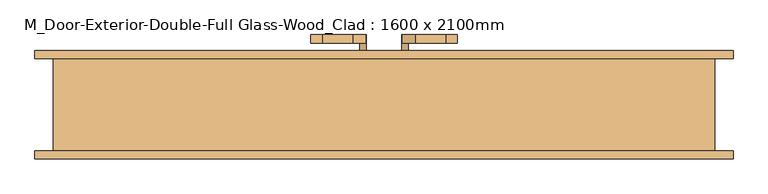
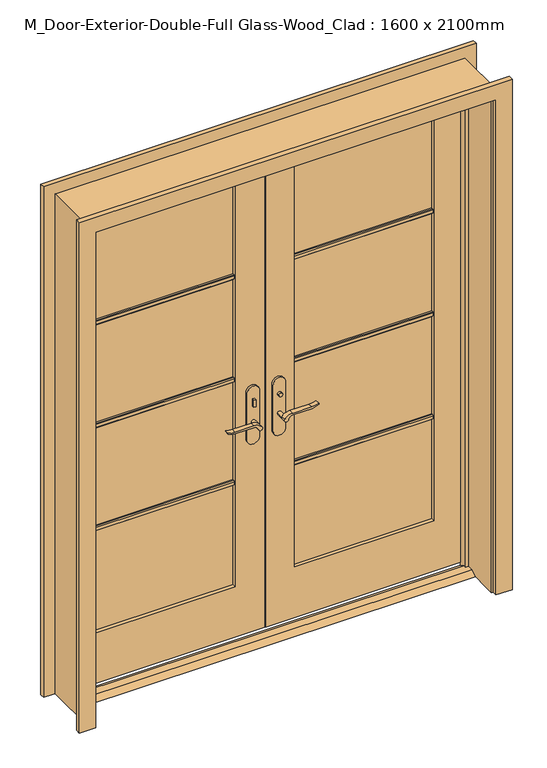
"""IFC4 building model written with IfcOpenShell, lengths in millimetres: door geometry, M_Door-Exterior-Double-Full Glass-Wood_Clad : 1600 x 2100mm."""

from ifc_helpers import new_model, si_unit, point, frame, frame_2d, origin, place, context, project, spatial, polyline, circle_curve, trimmed, segment, composite_curve, outline, extrude, faceted_brep, source, transform, mapped, element, save


def m_door_exterior_double_full_glass_wood_clad_1600_x_2100mm_56e3e291(model_context):
    return source(origin(), model_context, "Body", "SolidModel", [
        extrude(outline(polyline([(18.975, 15.0), (53.975, 15.0), (79.375, 0.0), (-6.425, 0.0), (18.975, 15.0)])), frame((-800.0, 0.0, 0.0), z_axis=(1.0, 0.0, 0.0), x_axis=(0.0, 1.0, 0.0)), (0.0, 0.0, 1.0), 1600.0),
        extrude(outline(polyline([(-47.4019111, 56.825), (-57.4019111, 56.825), (-57.4019111, 66.825), (-47.4019111, 66.825), (-47.4019111, 56.825)])), frame((0.0, 0.0, 981.9), z_axis=(0.0, 0.0, 1.0), x_axis=(1.0, 0.0, 0.0)), (0.0, 0.0, 1.0), 30.0),
        extrude(outline(composite_curve([segment(trimmed(circle_curve(frame_2d((996.9, -52.4019111)), 8.0), [point((996.9, -60.4019111))], [point((996.9, -44.4019111))], False, "CARTESIAN"), True, "CONTINUOUS"), segment(trimmed(circle_curve(frame_2d((996.9, -52.4019111)), 8.0), [point((996.9, -44.4019111))], [point((996.9, -60.4019111))], False, "CARTESIAN"), True, "CONTINUOUS")], self_intersect=False)), frame((0.0, 121.825, 0.0), z_axis=(0.0, 1.0, 0.0), x_axis=(0.0, 0.0, 1.0)), (0.0, 0.0, 1.0), 10.0),
        extrude(outline(composite_curve([segment(trimmed(circle_curve(frame_2d((897.1555521, -76.0694241)), 37.2832219), [point((919.0523287, -45.8937749))], [point((934.4, -77.7693445))], False, "CARTESIAN"), True, "CONTINUOUS"), segment(polyline([(934.4, -77.7693445), (934.4, -154.045502)]), True, "CONTINUOUS"), segment(trimmed(circle_curve(frame_2d((1017.6850638, -153.9791202)), 83.2850902), [point((934.4, -154.045502))], [point((939.4, -182.4019111))], True, "CARTESIAN"), True, "CONTINUOUS"), segment(polyline([(939.4, -182.4019111), (936.6135558, -182.4019111)]), True, "CONTINUOUS"), segment(trimmed(circle_curve(frame_2d((986.6709207, -150.4622499)), 59.3791355), [point((936.6135558, -182.4019111))], [point((927.4, -154.045502))], False, "CARTESIAN"), True, "CONTINUOUS"), segment(polyline([(927.4, -154.045502), (927.4, -77.7881013)]), True, "CONTINUOUS"), segment(trimmed(circle_curve(frame_2d((909.2738613, -77.7881013)), 18.1261387), [point((927.4, -77.7881013))], [point((914.4, -60.4019111))], True, "CARTESIAN"), True, "CONTINUOUS"), segment(trimmed(circle_curve(frame_2d((914.4, -52.4019111)), 8.0), [point((914.4, -60.4019111))], [point((919.0523287, -45.8937749))], False, "CARTESIAN"), True, "CONTINUOUS")], self_intersect=False)), frame((0.0, 16.825, 0.0), z_axis=(0.0, 1.0, 0.0), x_axis=(0.0, 0.0, 1.0)), (0.0, 0.0, 1.0), 20.0),
        extrude(outline(composite_curve([segment(trimmed(circle_curve(frame_2d((914.4, -52.4019111)), 8.0), [point((914.3999903, -60.4019111))], [point((919.0523287, -45.8937749))], False, "CARTESIAN"), True, "CONTINUOUS"), segment(trimmed(circle_curve(frame_2d((897.1555521, -76.0694241)), 37.2832219), [point((919.0523287, -45.8937749))], [point((934.4, -77.7693445))], False, "CARTESIAN"), True, "CONTINUOUS"), segment(polyline([(934.4, -77.7693445), (934.4, -154.045502)]), True, "CONTINUOUS"), segment(trimmed(circle_curve(frame_2d((1017.6850638, -153.9791202)), 83.2850902), [point((934.4, -154.045502))], [point((939.4, -182.4019111))], True, "CARTESIAN"), True, "CONTINUOUS"), segment(polyline([(939.4, -182.4019111), (936.6135558, -182.4019111)]), True, "CONTINUOUS"), segment(trimmed(circle_curve(frame_2d((986.6709207, -150.4622499)), 59.3791355), [point((936.6135558, -182.4019111))], [point((927.4, -154.045502))], False, "CARTESIAN"), True, "CONTINUOUS"), segment(polyline([(927.4, -154.045502), (927.4, -77.788099)]), True, "CONTINUOUS"), segment(trimmed(circle_curve(frame_2d((909.2738682, -77.788099)), 18.1261318), [point((927.4, -77.788099))], [point((914.3999903, -60.4019111))], True, "CARTESIAN"), True, "CONTINUOUS")], self_intersect=False)), frame((0.0, 151.825, 0.0), z_axis=(0.0, 1.0, 0.0), x_axis=(0.0, 0.0, 1.0)), (0.0, 0.0, 1.0), 20.0),
        extrude(outline(composite_curve([segment(trimmed(circle_curve(frame_2d((914.4, -52.4019111)), 8.0), [point((914.4, -60.4019111))], [point((914.4, -44.4019111))], False, "CARTESIAN"), True, "CONTINUOUS"), segment(trimmed(circle_curve(frame_2d((914.4, -52.4019111)), 8.0), [point((914.4, -44.4019111))], [point((914.4, -60.4019111))], False, "CARTESIAN"), True, "CONTINUOUS")], self_intersect=False)), frame((0.0, 36.825, 0.0), z_axis=(0.0, 1.0, 0.0), x_axis=(0.0, 0.0, 1.0)), (0.0, 0.0, 1.0), 30.0),
        extrude(outline(composite_curve([segment(trimmed(circle_curve(frame_2d((914.4, -52.4019111)), 8.0), [point((914.4, -60.4019111))], [point((914.4, -44.4019111))], False, "CARTESIAN"), True, "CONTINUOUS"), segment(trimmed(circle_curve(frame_2d((914.4, -52.4019111)), 8.0), [point((914.4, -44.4019111))], [point((914.4, -60.4019111))], False, "CARTESIAN"), True, "CONTINUOUS")], self_intersect=False)), frame((0.0, 121.825, 0.0), z_axis=(0.0, 1.0, 0.0), x_axis=(0.0, 0.0, 1.0)), (0.0, 0.0, 1.0), 30.0),
        extrude(outline(composite_curve([segment(polyline([(844.4, -27.4019111), (1039.4, -27.4019111)]), True, "CONTINUOUS"), segment(trimmed(circle_curve(frame_2d((1039.4, -52.4019111)), 25.0), [point((1039.4, -27.4019111))], [point((1039.4, -77.4019111))], False, "CARTESIAN"), True, "CONTINUOUS"), segment(polyline([(1039.4, -77.4019111), (844.4, -77.4019111)]), True, "CONTINUOUS"), segment(trimmed(circle_curve(frame_2d((844.4, -52.4019111)), 25.0), [point((844.4, -77.4019111))], [point((844.4, -27.4019111))], False, "CARTESIAN"), True, "CONTINUOUS")], self_intersect=False)), frame((0.0, 66.825, 0.0), z_axis=(0.0, 1.0, 0.0), x_axis=(0.0, 0.0, 1.0)), (0.0, 0.0, 1.0), 10.0),
        extrude(outline(composite_curve([segment(polyline([(844.4, -27.4019111), (1039.4, -27.4019111)]), True, "CONTINUOUS"), segment(trimmed(circle_curve(frame_2d((1039.4, -52.4019111)), 25.0), [point((1039.4, -27.4019111))], [point((1039.4, -77.4019111))], False, "CARTESIAN"), True, "CONTINUOUS"), segment(polyline([(1039.4, -77.4019111), (844.4, -77.4019111)]), True, "CONTINUOUS"), segment(trimmed(circle_curve(frame_2d((844.4, -52.4019111)), 25.0), [point((844.4, -77.4019111))], [point((844.4, -27.4019111))], False, "CARTESIAN"), True, "CONTINUOUS")], self_intersect=False)), frame((0.0, 111.825, 0.0), z_axis=(0.0, 1.0, 0.0), x_axis=(0.0, 0.0, 1.0)), (0.0, 0.0, 1.0), 10.0),
        extrude(outline(polyline([(47.3875, 131.825), (57.3875, 131.825), (57.3875, 121.825), (47.3875, 121.825), (47.3875, 131.825)])), frame((0.0, 0.0, 981.9), z_axis=(0.0, 0.0, 1.0), x_axis=(1.0, 0.0, 0.0)), (0.0, 0.0, 1.0), 30.0),
        extrude(outline(composite_curve([segment(trimmed(circle_curve(frame_2d((996.9, 52.3875)), 8.0), [point((996.9, 60.3875))], [point((996.9, 44.3875))], False, "CARTESIAN"), True, "CONTINUOUS"), segment(trimmed(circle_curve(frame_2d((996.9, 52.3875)), 8.0), [point((996.9, 44.3875))], [point((996.9, 60.3875))], False, "CARTESIAN"), True, "CONTINUOUS")], self_intersect=False)), frame((0.0, 56.825, 0.0), z_axis=(0.0, 1.0, 0.0), x_axis=(0.0, 0.0, 1.0)), (0.0, 0.0, 1.0), 10.0),
        extrude(outline(composite_curve([segment(trimmed(circle_curve(frame_2d((914.4, 52.3875)), 8.0), [point((919.0523287, 45.8793637))], [point((914.4, 60.3875))], False, "CARTESIAN"), True, "CONTINUOUS"), segment(trimmed(circle_curve(frame_2d((909.2738613, 77.7736901)), 18.1261387), [point((914.4, 60.3875))], [point((927.4, 77.7736901))], True, "CARTESIAN"), True, "CONTINUOUS"), segment(polyline([(927.4, 77.7736901), (927.4, 154.0310909)]), True, "CONTINUOUS"), segment(trimmed(circle_curve(frame_2d((986.6709207, 150.4478388)), 59.3791355), [point((927.4, 154.0310909))], [point((936.6135558, 182.3875))], False, "CARTESIAN"), True, "CONTINUOUS"), segment(polyline([(936.6135558, 182.3875), (939.4, 182.3875)]), True, "CONTINUOUS"), segment(trimmed(circle_curve(frame_2d((1017.6850638, 153.9647091)), 83.2850902), [point((939.4, 182.3875))], [point((934.4, 154.0310909))], True, "CARTESIAN"), True, "CONTINUOUS"), segment(polyline([(934.4, 154.0310909), (934.4, 77.7549333)]), True, "CONTINUOUS"), segment(trimmed(circle_curve(frame_2d((897.1555521, 76.0550129)), 37.2832219), [point((934.4, 77.7549333))], [point((919.0523287, 45.8793637))], False, "CARTESIAN"), True, "CONTINUOUS")], self_intersect=False)), frame((0.0, 151.825, 0.0), z_axis=(0.0, 1.0, 0.0), x_axis=(0.0, 0.0, 1.0)), (0.0, 0.0, 1.0), 20.0),
        extrude(outline(composite_curve([segment(trimmed(circle_curve(frame_2d((909.2738682, 77.7736878)), 18.1261318), [point((914.3999903, 60.3875))], [point((927.4, 77.7736878))], True, "CARTESIAN"), True, "CONTINUOUS"), segment(polyline([(927.4, 77.7736878), (927.4, 154.0310909)]), True, "CONTINUOUS"), segment(trimmed(circle_curve(frame_2d((986.6709207, 150.4478388)), 59.3791355), [point((927.4, 154.0310909))], [point((936.6135558, 182.3875))], False, "CARTESIAN"), True, "CONTINUOUS"), segment(polyline([(936.6135558, 182.3875), (939.4, 182.3875)]), True, "CONTINUOUS"), segment(trimmed(circle_curve(frame_2d((1017.6850638, 153.9647091)), 83.2850902), [point((939.4, 182.3875))], [point((934.4, 154.0310909))], True, "CARTESIAN"), True, "CONTINUOUS"), segment(polyline([(934.4, 154.0310909), (934.4, 77.7549333)]), True, "CONTINUOUS"), segment(trimmed(circle_curve(frame_2d((897.1555521, 76.0550129)), 37.2832219), [point((934.4, 77.7549333))], [point((919.0523287, 45.8793637))], False, "CARTESIAN"), True, "CONTINUOUS"), segment(trimmed(circle_curve(frame_2d((914.4, 52.3875)), 8.0), [point((919.0523287, 45.8793637))], [point((914.3999903, 60.3875))], False, "CARTESIAN"), True, "CONTINUOUS")], self_intersect=False)), frame((0.0, 16.825, 0.0), z_axis=(0.0, 1.0, 0.0), x_axis=(0.0, 0.0, 1.0)), (0.0, 0.0, 1.0), 20.0),
        extrude(outline(composite_curve([segment(trimmed(circle_curve(frame_2d((914.4, 52.3875)), 8.0), [point((914.4, 60.3875))], [point((914.4, 44.3875))], False, "CARTESIAN"), True, "CONTINUOUS"), segment(trimmed(circle_curve(frame_2d((914.4, 52.3875)), 8.0), [point((914.4, 44.3875))], [point((914.4, 60.3875))], False, "CARTESIAN"), True, "CONTINUOUS")], self_intersect=False)), frame((0.0, 121.825, 0.0), z_axis=(0.0, 1.0, 0.0), x_axis=(0.0, 0.0, 1.0)), (0.0, 0.0, 1.0), 30.0),
        extrude(outline(composite_curve([segment(trimmed(circle_curve(frame_2d((914.4, 52.3875)), 8.0), [point((914.4, 60.3875))], [point((914.4, 44.3875))], False, "CARTESIAN"), True, "CONTINUOUS"), segment(trimmed(circle_curve(frame_2d((914.4, 52.3875)), 8.0), [point((914.4, 44.3875))], [point((914.4, 60.3875))], False, "CARTESIAN"), True, "CONTINUOUS")], self_intersect=False)), frame((0.0, 36.825, 0.0), z_axis=(0.0, 1.0, 0.0), x_axis=(0.0, 0.0, 1.0)), (0.0, 0.0, 1.0), 30.0),
        extrude(outline(composite_curve([segment(trimmed(circle_curve(frame_2d((844.4, 52.3875)), 25.0), [point((844.4, 27.3875))], [point((844.4, 77.3875))], False, "CARTESIAN"), True, "CONTINUOUS"), segment(polyline([(844.4, 77.3875), (1039.4, 77.3875)]), True, "CONTINUOUS"), segment(trimmed(circle_curve(frame_2d((1039.4, 52.3875)), 25.0), [point((1039.4, 77.3875))], [point((1039.4, 27.3875))], False, "CARTESIAN"), True, "CONTINUOUS"), segment(polyline([(1039.4, 27.3875), (844.4, 27.3875)]), True, "CONTINUOUS")], self_intersect=False)), frame((0.0, 111.825, 0.0), z_axis=(0.0, 1.0, 0.0), x_axis=(0.0, 0.0, 1.0)), (0.0, 0.0, 1.0), 10.0),
        extrude(outline(composite_curve([segment(trimmed(circle_curve(frame_2d((844.4, 52.3875)), 25.0), [point((844.4, 27.3875))], [point((844.4, 77.3875))], False, "CARTESIAN"), True, "CONTINUOUS"), segment(polyline([(844.4, 77.3875), (1039.4, 77.3875)]), True, "CONTINUOUS"), segment(trimmed(circle_curve(frame_2d((1039.4, 52.3875)), 25.0), [point((1039.4, 77.3875))], [point((1039.4, 27.3875))], False, "CARTESIAN"), True, "CONTINUOUS"), segment(polyline([(1039.4, 27.3875), (844.4, 27.3875)]), True, "CONTINUOUS")], self_intersect=False)), frame((0.0, 66.825, 0.0), z_axis=(0.0, 1.0, 0.0), x_axis=(0.0, 0.0, 1.0)), (0.0, 0.0, 1.0), 10.0),
        extrude(outline(polyline([(90.825, 1552.025), (90.825, 1532.975), (84.475, 1532.975), (81.3, 1536.15), (81.3, 1548.85), (84.475, 1552.025), (90.825, 1552.025)])), frame((120.0, 0.0, 0.0), z_axis=(1.0, 0.0, 0.0), x_axis=(0.0, 1.0, 0.0)), (0.0, 0.0, 1.0), 560.0),
        extrude(outline(polyline([(90.825, 1114.525), (90.825, 1095.475), (84.475, 1095.475), (81.3, 1098.65), (81.3, 1111.35), (84.475, 1114.525), (90.825, 1114.525)])), frame((120.0, 0.0, 0.0), z_axis=(1.0, 0.0, 0.0), x_axis=(0.0, 1.0, 0.0)), (0.0, 0.0, 1.0), 560.0),
        extrude(outline(polyline([(90.825, 677.025), (90.825, 657.975), (84.475, 657.975), (81.3, 661.15), (81.3, 673.85), (84.475, 677.025), (90.825, 677.025)])), frame((120.0, 0.0, 0.0), z_axis=(1.0, 0.0, 0.0), x_axis=(0.0, 1.0, 0.0)), (0.0, 0.0, 1.0), 560.0),
        extrude(outline(polyline([(97.825, 1552.025), (104.175, 1552.025), (107.35, 1548.85), (107.35, 1536.15), (104.175, 1532.975), (97.825, 1532.975), (97.825, 1552.025)])), frame((-680.0, 0.0, 0.0), z_axis=(1.0, 0.0, 0.0), x_axis=(0.0, 1.0, 0.0)), (0.0, 0.0, 1.0), 560.0),
        extrude(outline(polyline([(97.825, 1114.525), (104.175, 1114.525), (107.35, 1111.35), (107.35, 1098.65), (104.175, 1095.475), (97.825, 1095.475), (97.825, 1114.525)])), frame((-680.0, 0.0, 0.0), z_axis=(1.0, 0.0, 0.0), x_axis=(0.0, 1.0, 0.0)), (0.0, 0.0, 1.0), 560.0),
        extrude(outline(polyline([(97.825, 677.025), (104.175, 677.025), (107.35, 673.85), (107.35, 661.15), (104.175, 657.975), (97.825, 657.975), (97.825, 677.025)])), frame((-680.0, 0.0, 0.0), z_axis=(1.0, 0.0, 0.0), x_axis=(0.0, 1.0, 0.0)), (0.0, 0.0, 1.0), 560.0),
        extrude(outline(polyline([(97.825, 1552.025), (104.175, 1552.025), (107.35, 1548.85), (107.35, 1536.15), (104.175, 1532.975), (97.825, 1532.975), (97.825, 1552.025)])), frame((120.0, 0.0, 0.0), z_axis=(1.0, 0.0, 0.0), x_axis=(0.0, 1.0, 0.0)), (0.0, 0.0, 1.0), 560.0),
        extrude(outline(polyline([(97.825, 1114.525), (104.175, 1114.525), (107.35, 1111.35), (107.35, 1098.65), (104.175, 1095.475), (97.825, 1095.475), (97.825, 1114.525)])), frame((120.0, 0.0, 0.0), z_axis=(1.0, 0.0, 0.0), x_axis=(0.0, 1.0, 0.0)), (0.0, 0.0, 1.0), 560.0),
        extrude(outline(polyline([(97.825, 677.025), (104.175, 677.025), (107.35, 673.85), (107.35, 661.15), (104.175, 657.975), (97.825, 657.975), (97.825, 677.025)])), frame((120.0, 0.0, 0.0), z_axis=(1.0, 0.0, 0.0), x_axis=(0.0, 1.0, 0.0)), (0.0, 0.0, 1.0), 560.0),
        extrude(outline(polyline([(90.825, 1552.025), (90.825, 1532.975), (84.475, 1532.975), (81.3, 1536.15), (81.3, 1548.85), (84.475, 1552.025), (90.825, 1552.025)])), frame((-680.0, 0.0, 0.0), z_axis=(1.0, 0.0, 0.0), x_axis=(0.0, 1.0, 0.0)), (0.0, 0.0, 1.0), 560.0),
        extrude(outline(polyline([(90.825, 1114.525), (90.825, 1095.475), (84.475, 1095.475), (81.3, 1098.65), (81.3, 1111.35), (84.475, 1114.525), (90.825, 1114.525)])), frame((-680.0, 0.0, 0.0), z_axis=(1.0, 0.0, 0.0), x_axis=(0.0, 1.0, 0.0)), (0.0, 0.0, 1.0), 560.0),
        extrude(outline(polyline([(90.825, 677.025), (90.825, 657.975), (84.475, 657.975), (81.3, 661.15), (81.3, 673.85), (84.475, 677.025), (90.825, 677.025)])), frame((-680.0, 0.0, 0.0), z_axis=(1.0, 0.0, 0.0), x_axis=(0.0, 1.0, 0.0)), (0.0, 0.0, 1.0), 560.0),
        extrude(outline(polyline([(0.0, 806.35), (0.0, 871.35), (2171.35, 871.35), (2171.35, -871.35), (0.0, -871.35), (0.0, -806.35), (2106.35, -806.35), (2106.35, 806.35), (0.0, 806.35)])), frame((0.0, 111.825, 0.0), z_axis=(0.0, 1.0, 0.0), x_axis=(0.0, 0.0, 1.0)), (0.0, 0.0, 1.0), 20.0),
        extrude(outline(polyline([(0.0, 806.35), (0.0, 871.35), (2171.35, 871.35), (2171.35, -871.35), (0.0, -871.35), (0.0, -806.35), (2106.35, -806.35), (2106.35, 806.35), (0.0, 806.35)])), frame((0.0, -138.175, 0.0), z_axis=(0.0, 1.0, 0.0), x_axis=(0.0, 0.0, 1.0)), (0.0, 0.0, 1.0), 20.0),
        extrude(outline(polyline([(15.0, 800.0), (2100.0, 800.0), (2100.0, 1.5875), (15.0, 1.5875), (15.0, 800.0)]), holes=[polyline([(1980.0, 120.0), (1980.0, 680.0), (230.0, 680.0), (230.0, 120.0), (1980.0, 120.0)])]), frame((0.0, 76.825, 0.0), z_axis=(0.0, 1.0, 0.0), x_axis=(0.0, 0.0, 1.0)), (0.0, 0.0, 1.0), 35.0),
        extrude(outline(polyline([(2100.0, -800.0), (15.0, -800.0), (15.0, -1.6019111), (2100.0, -1.6019111), (2100.0, -800.0)]), holes=[polyline([(230.0, -680.0), (1980.0, -680.0), (1980.0, -120.0), (230.0, -120.0), (230.0, -680.0)])]), frame((0.0, 76.825, 0.0), z_axis=(0.0, 1.0, 0.0), x_axis=(0.0, 0.0, 1.0)), (0.0, 0.0, 1.0), 35.0),
        faceted_brep([(825.0, 111.825, 0.0), (825.0, -118.175, 0.0), (800.0, -118.175, 0.0), (800.0, 41.9, 0.0), (787.3, 41.9, 0.0), (787.3, 76.825, 0.0), (800.0, 76.825, 0.0), (800.0, 111.825, 0.0), (825.0, 111.825, 2125.0), (825.0, -118.175, 2125.0), (-825.0, -118.175, 2125.0), (-825.0, -118.175, 0.0), (-800.0, -118.175, 0.0), (-800.0, -118.175, 2100.0), (800.0, -118.175, 2100.0), (800.0, 41.9, 2100.0), (-800.0, 41.9, 2100.0), (-800.0, 41.9, 0.0), (-787.3, 41.9, 0.0), (-787.3, 41.9, 2087.3), (787.3, 41.9, 2087.3), (787.3, 76.825, 2087.3), (1.5875, 76.825, 2087.3), (-1.6019111, 76.825, 2087.3), (-787.3, 76.825, 2087.3), (-787.3, 76.825, 0.0), (-800.0, 76.825, 0.0), (-800.0, 76.825, 2100.0), (-1.6019111, 76.825, 2100.0), (1.5875, 76.825, 2100.0), (800.0, 76.825, 2100.0), (800.0, 111.825, 2100.0), (1.5875, 111.825, 2100.0), (-1.6019111, 111.825, 2100.0), (-800.0, 111.825, 2100.0), (-800.0, 111.825, 0.0), (-825.0, 111.825, 0.0), (-825.0, 111.825, 2125.0)], [[[0, 1, 2, 3, 4, 5, 6, 7]], [[1, 0, 8, 9]], [[2, 1, 9, 10, 11, 12, 13, 14]], [[3, 2, 14, 15]], [[4, 3, 15, 16, 17, 18, 19, 20]], [[5, 4, 20, 21]], [[6, 5, 21, 22, 23, 24, 25, 26, 27, 28, 29, 30]], [[7, 6, 30, 31]], [[0, 7, 31, 32, 33, 34, 35, 36, 37, 8]], [[9, 8, 37, 10]], [[14, 13, 16, 15]], [[20, 19, 24, 23, 22, 21]], [[31, 30, 29, 28, 27, 34, 33, 32]], [[12, 11, 36, 35, 26, 25, 18, 17]], [[11, 10, 37, 36]], [[13, 12, 17, 16]], [[19, 18, 25, 24]], [[27, 26, 35, 34]]]),
        extrude(outline(polyline([(680.0, 90.825), (120.0, 90.825), (120.0, 97.825), (680.0, 97.825), (680.0, 90.825)])), frame((0.0, 0.0, 230.0), z_axis=(0.0, 0.0, 1.0), x_axis=(1.0, 0.0, 0.0)), (0.0, 0.0, 1.0), 1750.0),
        extrude(outline(polyline([(-120.0, 90.825), (-680.0, 90.825), (-680.0, 97.825), (-120.0, 97.825), (-120.0, 90.825)])), frame((0.0, 0.0, 230.0), z_axis=(0.0, 0.0, 1.0), x_axis=(1.0, 0.0, 0.0)), (0.0, 0.0, 1.0), 1750.0),
    ])


if __name__ == "__main__":
    model = new_model("IFC4")
    model_context = context("Model", 3, world=origin())
    ifc_project = project(units=[si_unit("LENGTHUNIT", "METRE", prefix="MILLI")], contexts=[model_context])
    site = spatial("IfcSite", under=ifc_project)
    building = spatial("IfcBuilding", under=site)
    placement = place(None, origin())
    m_door_exterior_double_full_glass_wood_clad_1600_x_2100mm_shape = m_door_exterior_double_full_glass_wood_clad_1600_x_2100mm_56e3e291(model_context)
    element("IfcDoor", 1, ObjectType="M_Door-Exterior-Double-Full Glass-Wood_Clad : 1600 x 2100mm", at=placement, inside=building, context=model_context, shape_type="MappedRepresentation", body=[
        mapped(m_door_exterior_double_full_glass_wood_clad_1600_x_2100mm_shape, transform((0.0, 0.0, 0.0), x_axis=(1.0, 0.0, 0.0), y_axis=(0.0, 1.0, 0.0), z_axis=(0.0, 0.0, 1.0))),
    ])
    save(model, "model.ifc")

# Revit data of these elements
# Type "M_Door-Exterior-Double-Full Glass-Wood_Clad : 1600 x 2100mm"
#   Type Mark = "41"
#   Assembly Code = "B2030100"
#   Analytic Construction = "French door, wood frame with double glass"
#   Top Rail = 12 cm
#   Threshold Offset [instance default] = 1.5 cm
#   Thickness = 3.5 cm
#   Thermal Resistance (R) = 0.337392 (m²·K)/W
#   Swing Angle [instance default] = 90.00°
#   Stiles = 12 cm
#   Rough Width = 165 cm
#   Rough Height = 212.5 cm
#   Panel Width = 80 cm
#   Door Offset [instance default] = 0 cm
#   Height = 210 cm
#   Width = 160 cm
#   Heat Transfer Coefficient (U) = 2.96405 W/(m²·K)
#   Bottom Rail = 23 cm
#   Exterior Trim [instance default] = yes
#   Threshold [instance default] = yes
#   Show Grill [instance default] = yes
#   Function = 1
#   Trim Material = Cherry
#   Threshold Material = Cherry
#   Panel Material = Cherry
#   Glazing = Glass
#   Frame Material = Cherry
#   Door Handle Material = Aluminum
#   Visual Light Transmittance = 0
#   Solar Heat Gain Coefficient = 0
#   Wall Closure = (empty or 0)
#   Construction Type = (empty or 0)
# Element 1 (IfcDoor, "M_Door-Exterior-Double-Full Glass-Wood_Clad : 1600 x 2100mm")
#   Materials on its faces: "Cherry", "Aluminum", "Glass"
# Materials
#   "Cherry": class "Wood", colour RGB 226 177 128, transparency 0, Description = "Prunus Serotina", Cost = 0
#   "Glass": class "Glass", colour RGB 0 128 192, transparency 0.9, Description = "Soda Lime Glass", Cost = 0
#   "Aluminum": class "Metal", colour RGB 247 247 247, transparency 0, Description = "Aluminum 6061", Cost = 0
